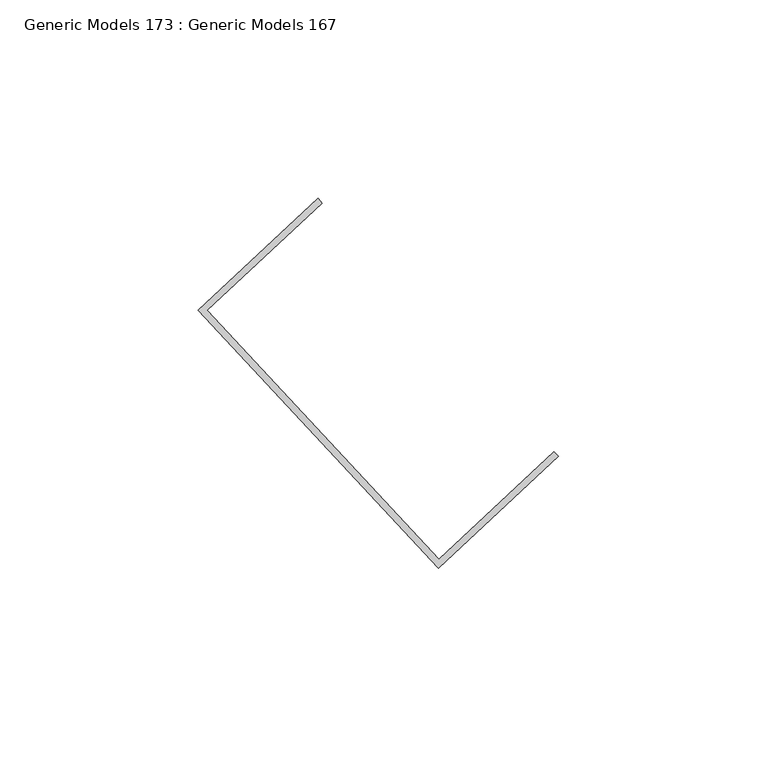
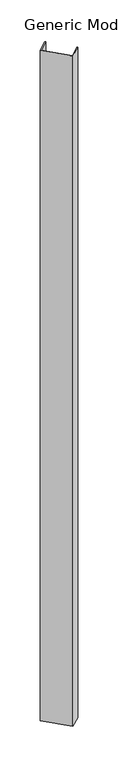
"""IFC4 building model written with IfcOpenShell, lengths in millimetres: proxy geometry, Generic Models 173 : Generic Models 167."""

from ifc_helpers import new_model, si_unit, origin, origin_with_axes, place, context, project, spatial, polyline, outline, extrude, source, transform, mapped, element, save


def generic_models_173_generic_models_167_0d7540df(model_context):
    return source(origin(), model_context, "Body", "SweptSolid", [
        extrude(outline(polyline([(59289.3941667, 4343.2668188), (59347.8584761, 4280.5715227), (59376.8840762, 4307.6383327), (59377.9667486, 4306.4773087), (59347.7801245, 4278.3278263), (59287.1504703, 4343.3451704), (59317.3370944, 4371.4946527), (59318.4197668, 4370.3336287), (59289.3941667, 4343.2668188)])), origin_with_axes(), (0.0, 0.0, 1.0), 2133.6),
    ])


if __name__ == "__main__":
    model = new_model("IFC4")
    model_context = context("Model", 3, world=origin())
    ifc_project = project(units=[si_unit("LENGTHUNIT", "METRE", prefix="MILLI")], contexts=[model_context])
    site = spatial("IfcSite", under=ifc_project)
    building = spatial("IfcBuilding", under=site)
    placement = place(None, origin())
    generic_models_173_generic_models_167_shape = generic_models_173_generic_models_167_0d7540df(model_context)
    element("IfcBuildingElementProxy", 1, Name="Generic Models 173 : Generic Models 167", ObjectType="Generic Models 173 : Generic Models 167", at=placement, inside=building, context=model_context, shape_type="MappedRepresentation", body=[
        mapped(generic_models_173_generic_models_167_shape, transform((0.0, 0.0, 0.0), x_axis=(1.0, 0.0, 0.0), y_axis=(0.0, 1.0, 0.0), z_axis=(0.0, 0.0, 1.0))),
    ])
    save(model, "model.ifc")

# Revit data of these elements
# Element 1 (IfcBuildingElementProxy, "Generic Models 173 : Generic Models 167")
#   Materials on its faces: "EXISTING STOREFRONT"
# Materials
#   "EXISTING STOREFRONT": class "Metal", colour RGB 244 244 244, transparency 0, Description = "Aluminum 6061", Cost = 0
